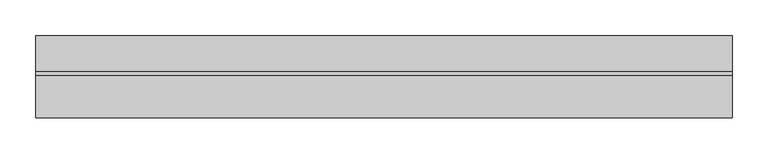
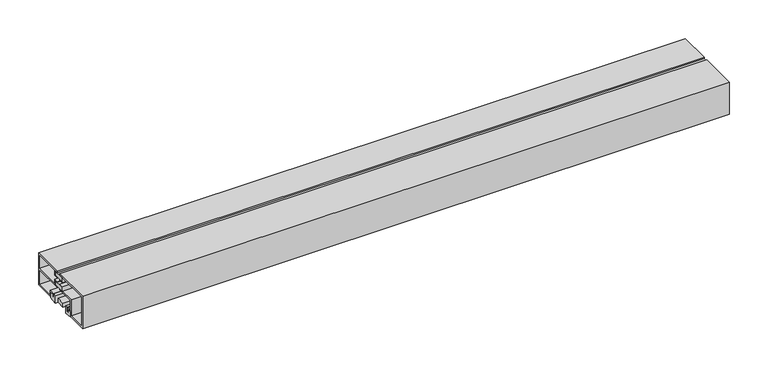
"""IFC4 building model written with IfcOpenShell, lengths in millimetres: proxy geometry, Generic Models 3:Generic Models 1:4:Generic Models 1:4 : Generic Models 3:Generic Models 1:300625:338780:Generic Models 1:4:Generic Models 1:4 : Generic Models 3:Generic Models 1:300625:338780 : Generic Models 3:Generic Models 1:4:Generic Models 1:4 : Generic Models 3:Generic Models 1:300625:338780:3 : Generic Models 3:Generic Models 1:4:Generic Models 1:4 : Generic Models 3:Generic Models 1:300625:338780:Generic Models 1:4:Generic Models 1:4 : Generic Models 3:Generic Models 1:300625:338780 : Generic Models 3:Generic Models 1:4:Generic Models 1:4 : Generic Models 3:Generic Models 1:300625:338780:301383."""

from ifc_helpers import new_model, si_unit, frame, origin, place, context, project, spatial, polyline, outline, extrude, source, transform, mapped, element, save


def generic_models_5c43024b(model_context):
    return source(origin(), model_context, "Body", "SweptSolid", [
        extrude(outline(polyline([(570446.2867239, -579047.9760005), (570446.2867239, -579064.0874367), (569476.3242239, -579064.0874367), (569476.3242239, -579047.9760005), (570446.2867239, -579047.9760005)])), frame((0.0, 0.0, 3693.6142952), z_axis=(0.0, 0.0, 1.0), x_axis=(1.0, 0.0, 0.0)), (0.0, 0.0, 1.0), 6.0797872),
        extrude(outline(polyline([(570446.2867239, -579047.8857325), (570446.2867239, -579063.9971687), (569476.3242239, -579063.9971687), (569476.3242239, -579047.8857325), (570446.2867239, -579047.8857325)])), frame((0.0, 0.0, 3678.5668218), z_axis=(0.0, 0.0, 1.0), x_axis=(1.0, 0.0, 0.0)), (0.0, 0.0, 1.0), 6.0797872),
        extrude(outline(polyline([(570446.2867239, -579054.6832724), (570446.2867239, -579067.3832724), (569476.3242239, -579067.3832724), (569476.3242239, -579054.6832724), (570446.2867239, -579054.6832724)])), frame((0.0, 0.0, 3654.1359064), z_axis=(0.0, 0.0, 1.0), x_axis=(1.0, 0.0, 0.0)), (0.0, 0.0, 1.0), 6.3435484),
        extrude(outline(polyline([(-579086.0195091, 3650.2669395), (-579086.0195091, 3658.1066489), (-579081.7214373, 3658.1066489), (-579081.7214373, 3655.1627892), (-579078.8757591, 3655.1627892), (-579078.8757591, 3660.8763298), (-579074.1217032, 3660.8763298), (-579074.1217032, 3648.8060727), (-579086.0195091, 3650.2669395)])), frame((569476.3242239, 0.0, 0.0), z_axis=(1.0, 0.0, 0.0), x_axis=(0.0, 1.0, 0.0)), (0.0, 0.0, 1.0), 969.9625),
        extrude(outline(polyline([(-579043.1907857, 3655.1627892), (-579040.3451075, 3655.1627892), (-579040.3451075, 3658.1066489), (-579036.0470357, 3658.1066489), (-579036.0470357, 3650.2669395), (-579047.9448415, 3648.8060727), (-579047.9448415, 3660.8763298), (-579043.1907857, 3660.8763298), (-579043.1907857, 3655.1627892)])), frame((569476.3242239, 0.0, 0.0), z_axis=(1.0, 0.0, 0.0), x_axis=(0.0, 1.0, 0.0)), (0.0, 0.0, 1.0), 969.9625),
        extrude(outline(polyline([(-579003.8663841, 3651.2837766), (-579035.6501607, 3651.2837766), (-579035.6501607, 3658.5035239), (-579040.7419825, 3658.5035239), (-579040.7419825, 3655.5596642), (-579042.7939107, 3655.5596642), (-579042.7939107, 3660.4794548), (-579033.7502272, 3660.4794548), (-579033.7502272, 3653.1935757), (-579005.8423149, 3653.1935757), (-579005.8423149, 3676.6668883), (-579052.7495623, 3676.6668883), (-579052.7495623, 3678.5668218), (-579047.8857325, 3678.5668218), (-579047.8857325, 3684.646609), (-579052.7495623, 3684.646609), (-579052.7495623, 3685.9385638), (-579045.985799, 3685.9385638), (-579045.985799, 3678.5668218), (-579005.8423149, 3678.5668218), (-579005.8423149, 3700.1277874), (-579046.076067, 3700.1277874), (-579046.076067, 3692.3223404), (-579052.8398303, 3692.3223404), (-579052.8398303, 3693.6142952), (-579047.9760005, 3693.6142952), (-579047.9760005, 3699.6940824), (-579052.8398303, 3699.6940824), (-579052.8398303, 3702.05), (-579003.8663841, 3702.05), (-579003.8663841, 3651.2837766)])), frame((569476.3242239, 0.0, 0.0), z_axis=(1.0, 0.0, 0.0), x_axis=(0.0, 1.0, 0.0)), (0.0, 0.0, 1.0), 969.9625),
        extrude(outline(polyline([(-579081.3245623, 3658.5035239), (-579086.4163841, 3658.5035239), (-579086.4163841, 3651.2837766), (-579118.1663841, 3651.2837766), (-579118.1663841, 3702.05), (-579059.2236069, 3702.05), (-579059.2236069, 3699.6940824), (-579064.0874367, 3699.6940824), (-579064.0874367, 3693.6142952), (-579059.2236069, 3693.6142952), (-579059.2236069, 3692.3223404), (-579065.9873702, 3692.3223404), (-579065.9873702, 3700.1500665), (-579115.6584719, 3700.1500665), (-579115.6584719, 3653.1837101), (-579088.3163176, 3653.1837101), (-579088.3163176, 3678.5668218), (-579065.8971022, 3678.5668218), (-579065.8971022, 3685.9385638), (-579059.1333389, 3685.9385638), (-579059.1333389, 3684.646609), (-579063.9971687, 3684.646609), (-579063.9971687, 3678.5668218), (-579059.1333389, 3678.5668218), (-579059.1333389, 3676.6668883), (-579086.4163841, 3676.6668883), (-579086.4163841, 3660.4794548), (-579079.2726341, 3660.4794548), (-579079.2726341, 3655.5596642), (-579081.3245623, 3655.5596642), (-579081.3245623, 3658.5035239)])), frame((569476.3242239, 0.0, 0.0), z_axis=(1.0, 0.0, 0.0), x_axis=(0.0, 1.0, 0.0)), (0.0, 0.0, 1.0), 969.9625),
    ])


if __name__ == "__main__":
    model = new_model("IFC4")
    model_context = context("Model", 3, world=origin())
    ifc_project = project(units=[si_unit("LENGTHUNIT", "METRE", prefix="MILLI")], contexts=[model_context])
    site = spatial("IfcSite", under=ifc_project)
    building = spatial("IfcBuilding", under=site)
    placement = place(None, origin())
    generic_models_shape = generic_models_5c43024b(model_context)
    element("IfcBuildingElementProxy", 1, Name="Generic Models 3:Generic Models 1:4:Generic Models 1:4 : Generic Models 3:Generic Models 1:300625:338780:Generic Models 1:4:Generic Models 1:4 : Generic Models 3:Generic Models 1:300625:338780 : Generic Models 3:Generic Models 1:4:Generic Models 1:4 : Generic Models 3:Generic Models 1:300625:338780:3 : Generic Models 3:Generic Models 1:4:Generic Models 1:4 : Generic Models 3:Generic Models 1:300625:338780:Generic Models 1:4:Generic Models 1:4 : Generic Models 3:Generic Models 1:300625:338780 : Generic Models 3:Generic Models 1:4:Generic Models 1:4 : Generic Models 3:Generic Models 1:300625:338780:301383", ObjectType="Generic Models 3:Generic Models 1:4:Generic Models 1:4 : Generic Models 3:Generic Models 1:300625:338780:Generic Models 1:4:Generic Models 1:4 : Generic Models 3:Generic Models 1:300625:338780 : Generic Models 3:Generic Models 1:4:Generic Models 1:4 : Generic Models 3:Generic Models 1:300625:338780:3 : Generic Models 3:Generic Models 1:4:Generic Models 1:4 : Generic Models 3:Generic Models 1:300625:338780:Generic Models 1:4:Generic Models 1:4 : Generic Models 3:Generic Models 1:300625:338780 : Generic Models 3:Generic Models 1:4:Generic Models 1:4 : Generic Models 3:Generic Models 1:300625:338780:301383", at=placement, inside=building, context=model_context, shape_type="MappedRepresentation", body=[
        mapped(generic_models_shape, transform((0.0, 0.0, 0.0), x_axis=(1.0, 0.0, 0.0), y_axis=(0.0, 1.0, 0.0), z_axis=(0.0, 0.0, 1.0))),
    ])
    save(model, "model.ifc")

# Revit data of these elements
# Type "Generic Models 3:Generic Models 1:4:Generic Models 1:4 : Generic Models 3:Generic Models 1:300625:338780:Generic Models 1:4:Generic Models 1:4 : Generic Models 3:Generic Models 1:300625:338780 : Generic Models 3:Generic Models 1:4:Generic Models 1:4 : Generic Models 3:Generic Models 1:300625:338780:3 : Generic Models 3:Generic Models 1:4:Generic Models 1:4 : Generic Models 3:Generic Models 1:300625:338780:Generic Models 1:4:Generic Models 1:4 : Generic Models 3:Generic Models 1:300625:338780 : Generic Models 3:Generic Models 1:4:Generic Models 1:4 : Generic Models 3:Generic Models 1:300625:338780:301383"
#   NameOverride = "Generic Models 3:Generic Models 1:4:Generic Models 1:4 : Generic Models 3:Generic Models 1:300625:338780:Generic Models 1:4:Generic Models 1:4 : Generic Models 3:Generic Models 1:300625:338780 : Generic Models 3:Generic Models 1:4:Generic Models 1:4 : Generic Models 3:Generic Models 1:300625:338780:301383"
#   ObjectTypeOverride = "Generic Models 1:4:Generic Models 1:4 : Generic Models 3:Generic Models 1:300625:338780 : Generic Models 3:Generic Models 1:4:Generic Models 1:4 : Generic Models 3:Generic Models 1:300625:338780"
#   Reference = "Generic Models 1"
#   Tag = "301383"
# Element 1 (IfcBuildingElementProxy, "Generic Models 3:Generic Models 1:4:Generic Models 1:4 : Generic Models 3:Generic Models 1:300625:338780:Generic Models 1:4:Generic Models 1:4 : Generic Models 3:Generic Models 1:300625:338780 : Generic Models 3:Generic Models 1:4:Generic Models 1:4 : Generic Models 3:Generic Models 1:300625:338780:3 : Generic Models 3:Generic Models 1:4:Generic Models 1:4 : Generic Models 3:Generic Models 1:300625:338780:Generic Models 1:4:Generic Models 1:4 : Generic Models 3:Generic Models 1:300625:338780 : Generic Models 3:Generic Models 1:4:Generic Models 1:4 : Generic Models 3:Generic Models 1:300625:338780:301383")
#   Materials on its faces: "THERMAL BROKEN ALUMINUM STOREFRONT"
# Materials
#   "THERMAL BROKEN ALUMINUM STOREFRONT": class "Unassigned", colour RGB 244 244 244, transparency 0, Cost = 0
